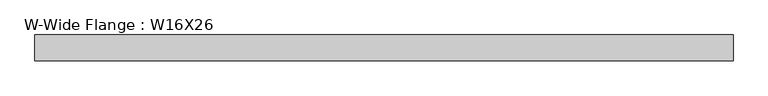
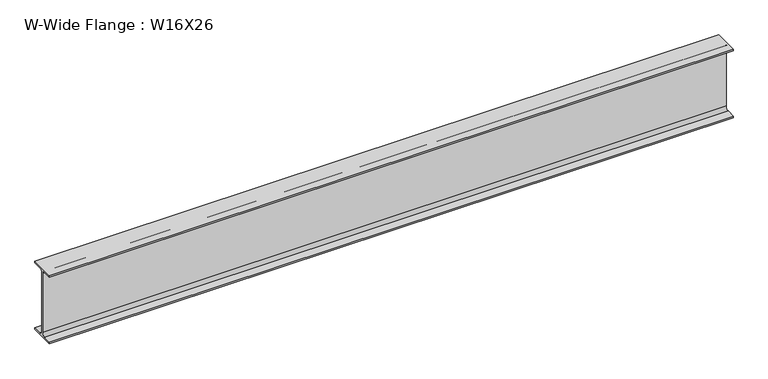
"""IFC4 building model written with IfcOpenShell, lengths in millimetres: beam geometry, W-Wide Flange : W16X26."""

from ifc_helpers import new_model, si_unit, point, frame, frame_2d, origin, place, context, project, spatial, polyline, circle_curve, trimmed, segment, composite_curve, outline, extrude, source, transform, mapped, element, save


def w_wide_flange_w16x26_d3a9b0fe(model_context):
    return source(origin(), model_context, "Body", "SweptSolid", [
        extrude(outline(composite_curve([segment(polyline([(69.85, -190.627), (69.85, -199.39), (-69.85, -199.39), (-69.85, -190.627), (-21.3995, -190.627)]), True, "CONTINUOUS"), segment(trimmed(circle_curve(frame_2d((-21.3995, -172.4025)), 18.2245), [point((-21.3995, -190.627))], [point((-3.175, -172.4025))], True, "CARTESIAN"), True, "CONTINUOUS"), segment(polyline([(-3.175, -172.4025), (-3.175, 172.4025)]), True, "CONTINUOUS"), segment(trimmed(circle_curve(frame_2d((-21.3995, 172.4025)), 18.2245), [point((-3.175, 172.4025))], [point((-21.3995, 190.627))], True, "CARTESIAN"), True, "CONTINUOUS"), segment(polyline([(-21.3995, 190.627), (-69.85, 190.627), (-69.85, 199.39), (69.85, 199.39), (69.85, 190.627), (21.3995, 190.627)]), True, "CONTINUOUS"), segment(trimmed(circle_curve(frame_2d((21.3995, 172.4025)), 18.2245), [point((21.3995, 190.627))], [point((3.175, 172.4025))], True, "CARTESIAN"), True, "CONTINUOUS"), segment(polyline([(3.175, 172.4025), (3.175, -172.4025)]), True, "CONTINUOUS"), segment(trimmed(circle_curve(frame_2d((21.3995, -172.4025)), 18.2245), [point((3.175, -172.4025))], [point((21.3995, -190.627))], True, "CARTESIAN"), True, "CONTINUOUS"), segment(polyline([(21.3995, -190.627), (69.85, -190.627)]), True, "CONTINUOUS")], self_intersect=False)), frame((-1892.3, 0.0, 0.0), z_axis=(1.0, 0.0, 0.0), x_axis=(0.0, 1.0, 0.0)), (0.0, 0.0, 1.0), 3784.6),
    ])


if __name__ == "__main__":
    model = new_model("IFC4")
    model_context = context("Model", 3, world=origin())
    ifc_project = project(units=[si_unit("LENGTHUNIT", "METRE", prefix="MILLI")], contexts=[model_context])
    site = spatial("IfcSite", under=ifc_project)
    building = spatial("IfcBuilding", under=site)
    placement = place(None, origin())
    w_wide_flange_w16x26_shape = w_wide_flange_w16x26_d3a9b0fe(model_context)
    element("IfcBeam", 1, ObjectType="W-Wide Flange : W16X26", at=placement, inside=building, context=model_context, shape_type="MappedRepresentation", body=[
        mapped(w_wide_flange_w16x26_shape, transform((0.0, 0.0, 0.0), x_axis=(1.0, 0.0, 0.0), y_axis=(0.0, 1.0, 0.0), z_axis=(0.0, 0.0, 1.0))),
    ])
    save(model, "model.ifc")

# Revit data of these elements
# Type "W-Wide Flange : W16X26"
#   Assembly Code = "B10"
#   W = 26
#   Length [instance default] = 5' - 0"
#   bf = 0' - 5 1/2"
#   d = 1' - 3.7"
#   k = 0' - 1 1/16"
#   k2 = 0' - 0.7175"
#   tf = 0' - 0.345"
#   tw = 0' - 0 1/4"
#   A = 0.0533333 SF
#   Structural Material [instance default] = Steel ASTM A992
# Element 1 (IfcBeam, "W-Wide Flange : W16X26")
#   Materials on its faces: "Steel ASTM A992"
# Materials
#   "Steel ASTM A992": class "Metal", colour RGB 199 199 199, transparency 0, Description = "Structural steel 50ksi", Cost = 0
